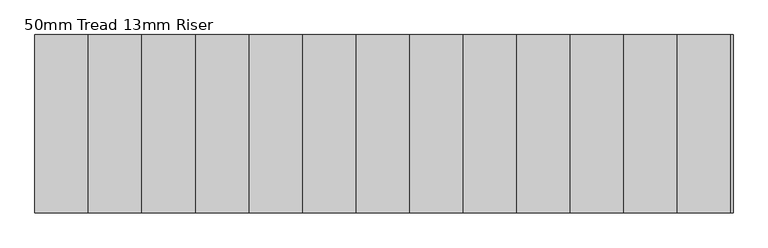
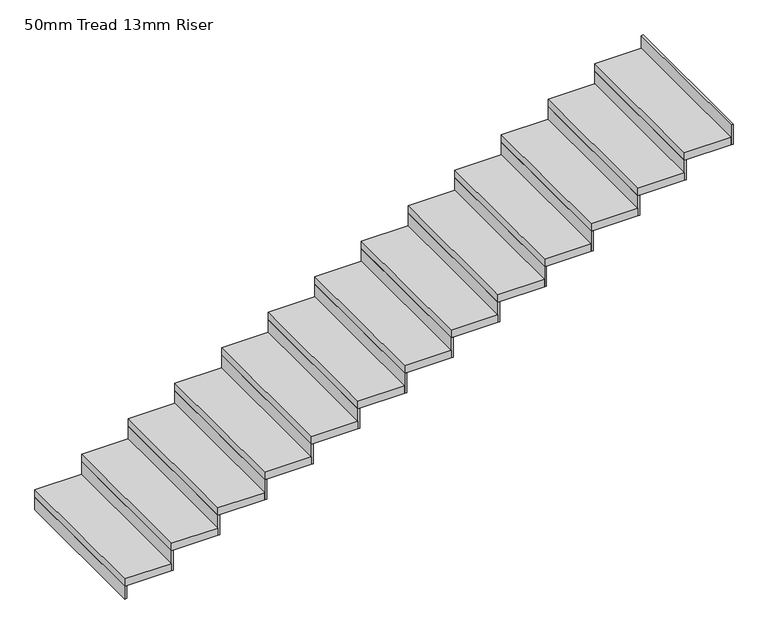
"""IFC4 building model written with IfcOpenShell, lengths in millimetres: stair flight geometry, 50mm Tread 13mm Riser."""

from ifc_helpers import new_model, si_unit, frame, origin, origin_with_axes, place, context, project, spatial, polyline, outline, extrude, source, transform, mapped, element, save


def stair_flight_50mm_tread_13mm_riser_4b704193(model_context):
    return source(origin(), model_context, "Body", "SweptSolid", [
        extrude(outline(polyline([(17862.336337, -4576.2808257), (17849.836337, -4576.2808257), (17849.836337, -3576.2808257), (17862.336337, -3576.2808257), (17862.336337, -4576.2808257)])), origin_with_axes(), (0.0, 0.0, 1.0), 86.3636364),
        extrude(outline(polyline([(18149.836337, -3576.2808257), (18149.836337, -4576.2808257), (17849.836337, -4576.2808257), (17849.836337, -3576.2808257), (18149.836337, -3576.2808257)])), frame((0.0, 0.0, 86.3636364), z_axis=(0.0, 0.0, 1.0), x_axis=(1.0, 0.0, 0.0)), (0.0, 0.0, 1.0), 50.0),
        extrude(outline(polyline([(18162.336337, -4576.2808257), (18149.836337, -4576.2808257), (18149.836337, -3576.2808257), (18162.336337, -3576.2808257), (18162.336337, -4576.2808257)])), frame((0.0, 0.0, 86.3636364), z_axis=(0.0, 0.0, 1.0), x_axis=(1.0, 0.0, 0.0)), (0.0, 0.0, 1.0), 136.3636364),
        extrude(outline(polyline([(18449.836337, -3576.2808257), (18449.836337, -4576.2808257), (18149.836337, -4576.2808257), (18149.836337, -3576.2808257), (18449.836337, -3576.2808257)])), frame((0.0, 0.0, 222.7272727), z_axis=(0.0, 0.0, 1.0), x_axis=(1.0, 0.0, 0.0)), (0.0, 0.0, 1.0), 50.0),
        extrude(outline(polyline([(18462.336337, -4576.2808257), (18449.836337, -4576.2808257), (18449.836337, -3576.2808257), (18462.336337, -3576.2808257), (18462.336337, -4576.2808257)])), frame((0.0, 0.0, 222.7272727), z_axis=(0.0, 0.0, 1.0), x_axis=(1.0, 0.0, 0.0)), (0.0, 0.0, 1.0), 136.3636364),
        extrude(outline(polyline([(18749.836337, -3576.2808257), (18749.836337, -4576.2808257), (18449.836337, -4576.2808257), (18449.836337, -3576.2808257), (18749.836337, -3576.2808257)])), frame((0.0, 0.0, 359.0909091), z_axis=(0.0, 0.0, 1.0), x_axis=(1.0, 0.0, 0.0)), (0.0, 0.0, 1.0), 50.0),
        extrude(outline(polyline([(18762.336337, -4576.2808257), (18749.836337, -4576.2808257), (18749.836337, -3576.2808257), (18762.336337, -3576.2808257), (18762.336337, -4576.2808257)])), frame((0.0, 0.0, 359.0909091), z_axis=(0.0, 0.0, 1.0), x_axis=(1.0, 0.0, 0.0)), (0.0, 0.0, 1.0), 136.3636364),
        extrude(outline(polyline([(19049.836337, -3576.2808257), (19049.836337, -4576.2808257), (18749.836337, -4576.2808257), (18749.836337, -3576.2808257), (19049.836337, -3576.2808257)])), frame((0.0, 0.0, 495.4545455), z_axis=(0.0, 0.0, 1.0), x_axis=(1.0, 0.0, 0.0)), (0.0, 0.0, 1.0), 50.0),
        extrude(outline(polyline([(19062.336337, -4576.2808257), (19049.836337, -4576.2808257), (19049.836337, -3576.2808257), (19062.336337, -3576.2808257), (19062.336337, -4576.2808257)])), frame((0.0, 0.0, 495.4545455), z_axis=(0.0, 0.0, 1.0), x_axis=(1.0, 0.0, 0.0)), (0.0, 0.0, 1.0), 136.3636364),
        extrude(outline(polyline([(19349.836337, -3576.2808257), (19349.836337, -4576.2808257), (19049.836337, -4576.2808257), (19049.836337, -3576.2808257), (19349.836337, -3576.2808257)])), frame((0.0, 0.0, 631.8181818), z_axis=(0.0, 0.0, 1.0), x_axis=(1.0, 0.0, 0.0)), (0.0, 0.0, 1.0), 50.0),
        extrude(outline(polyline([(19362.336337, -4576.2808257), (19349.836337, -4576.2808257), (19349.836337, -3576.2808257), (19362.336337, -3576.2808257), (19362.336337, -4576.2808257)])), frame((0.0, 0.0, 631.8181818), z_axis=(0.0, 0.0, 1.0), x_axis=(1.0, 0.0, 0.0)), (0.0, 0.0, 1.0), 136.3636364),
        extrude(outline(polyline([(19649.836337, -3576.2808257), (19649.836337, -4576.2808257), (19349.836337, -4576.2808257), (19349.836337, -3576.2808257), (19649.836337, -3576.2808257)])), frame((0.0, 0.0, 768.1818182), z_axis=(0.0, 0.0, 1.0), x_axis=(1.0, 0.0, 0.0)), (0.0, 0.0, 1.0), 50.0),
        extrude(outline(polyline([(19662.336337, -4576.2808257), (19649.836337, -4576.2808257), (19649.836337, -3576.2808257), (19662.336337, -3576.2808257), (19662.336337, -4576.2808257)])), frame((0.0, 0.0, 768.1818182), z_axis=(0.0, 0.0, 1.0), x_axis=(1.0, 0.0, 0.0)), (0.0, 0.0, 1.0), 136.3636364),
        extrude(outline(polyline([(19949.836337, -3576.2808257), (19949.836337, -4576.2808257), (19649.836337, -4576.2808257), (19649.836337, -3576.2808257), (19949.836337, -3576.2808257)])), frame((0.0, 0.0, 904.5454545), z_axis=(0.0, 0.0, 1.0), x_axis=(1.0, 0.0, 0.0)), (0.0, 0.0, 1.0), 50.0),
        extrude(outline(polyline([(19962.336337, -4576.2808257), (19949.836337, -4576.2808257), (19949.836337, -3576.2808257), (19962.336337, -3576.2808257), (19962.336337, -4576.2808257)])), frame((0.0, 0.0, 904.5454545), z_axis=(0.0, 0.0, 1.0), x_axis=(1.0, 0.0, 0.0)), (0.0, 0.0, 1.0), 136.3636364),
        extrude(outline(polyline([(20249.836337, -3576.2808257), (20249.836337, -4576.2808257), (19949.836337, -4576.2808257), (19949.836337, -3576.2808257), (20249.836337, -3576.2808257)])), frame((0.0, 0.0, 1040.9090909), z_axis=(0.0, 0.0, 1.0), x_axis=(1.0, 0.0, 0.0)), (0.0, 0.0, 1.0), 50.0),
        extrude(outline(polyline([(20262.336337, -4576.2808257), (20249.836337, -4576.2808257), (20249.836337, -3576.2808257), (20262.336337, -3576.2808257), (20262.336337, -4576.2808257)])), frame((0.0, 0.0, 1040.9090909), z_axis=(0.0, 0.0, 1.0), x_axis=(1.0, 0.0, 0.0)), (0.0, 0.0, 1.0), 136.3636364),
        extrude(outline(polyline([(20549.836337, -3576.2808257), (20549.836337, -4576.2808257), (20249.836337, -4576.2808257), (20249.836337, -3576.2808257), (20549.836337, -3576.2808257)])), frame((0.0, 0.0, 1177.2727273), z_axis=(0.0, 0.0, 1.0), x_axis=(1.0, 0.0, 0.0)), (0.0, 0.0, 1.0), 50.0),
        extrude(outline(polyline([(20562.336337, -4576.2808257), (20549.836337, -4576.2808257), (20549.836337, -3576.2808257), (20562.336337, -3576.2808257), (20562.336337, -4576.2808257)])), frame((0.0, 0.0, 1177.2727273), z_axis=(0.0, 0.0, 1.0), x_axis=(1.0, 0.0, 0.0)), (0.0, 0.0, 1.0), 136.3636364),
        extrude(outline(polyline([(20849.836337, -3576.2808257), (20849.836337, -4576.2808257), (20549.836337, -4576.2808257), (20549.836337, -3576.2808257), (20849.836337, -3576.2808257)])), frame((0.0, 0.0, 1313.6363636), z_axis=(0.0, 0.0, 1.0), x_axis=(1.0, 0.0, 0.0)), (0.0, 0.0, 1.0), 50.0),
        extrude(outline(polyline([(20862.336337, -4576.2808257), (20849.836337, -4576.2808257), (20849.836337, -3576.2808257), (20862.336337, -3576.2808257), (20862.336337, -4576.2808257)])), frame((0.0, 0.0, 1313.6363636), z_axis=(0.0, 0.0, 1.0), x_axis=(1.0, 0.0, 0.0)), (0.0, 0.0, 1.0), 136.3636364),
        extrude(outline(polyline([(21149.836337, -3576.2808257), (21149.836337, -4576.2808257), (20849.836337, -4576.2808257), (20849.836337, -3576.2808257), (21149.836337, -3576.2808257)])), frame((0.0, 0.0, 1450.0), z_axis=(0.0, 0.0, 1.0), x_axis=(1.0, 0.0, 0.0)), (0.0, 0.0, 1.0), 50.0),
        extrude(outline(polyline([(21162.336337, -4576.2808257), (21149.836337, -4576.2808257), (21149.836337, -3576.2808257), (21162.336337, -3576.2808257), (21162.336337, -4576.2808257)])), frame((0.0, 0.0, 1450.0), z_axis=(0.0, 0.0, 1.0), x_axis=(1.0, 0.0, 0.0)), (0.0, 0.0, 1.0), 136.3636364),
        extrude(outline(polyline([(21449.836337, -3576.2808257), (21449.836337, -4576.2808257), (21149.836337, -4576.2808257), (21149.836337, -3576.2808257), (21449.836337, -3576.2808257)])), frame((0.0, 0.0, 1586.3636364), z_axis=(0.0, 0.0, 1.0), x_axis=(1.0, 0.0, 0.0)), (0.0, 0.0, 1.0), 50.0),
        extrude(outline(polyline([(21462.336337, -4576.2808257), (21449.836337, -4576.2808257), (21449.836337, -3576.2808257), (21462.336337, -3576.2808257), (21462.336337, -4576.2808257)])), frame((0.0, 0.0, 1586.3636364), z_axis=(0.0, 0.0, 1.0), x_axis=(1.0, 0.0, 0.0)), (0.0, 0.0, 1.0), 136.3636364),
        extrude(outline(polyline([(21762.336337, -4576.2808257), (21749.836337, -4576.2808257), (21749.836337, -3576.2808257), (21762.336337, -3576.2808257), (21762.336337, -4576.2808257)])), frame((0.0, 0.0, 1722.7272727), z_axis=(0.0, 0.0, 1.0), x_axis=(1.0, 0.0, 0.0)), (0.0, 0.0, 1.0), 136.3636364),
        extrude(outline(polyline([(21749.836337, -3576.2808257), (21749.836337, -4576.2808257), (21449.836337, -4576.2808257), (21449.836337, -3576.2808257), (21749.836337, -3576.2808257)])), frame((0.0, 0.0, 1722.7272727), z_axis=(0.0, 0.0, 1.0), x_axis=(1.0, 0.0, 0.0)), (0.0, 0.0, 1.0), 50.0),
    ])


if __name__ == "__main__":
    model = new_model("IFC4")
    model_context = context("Model", 3, world=origin())
    ifc_project = project(units=[si_unit("LENGTHUNIT", "METRE", prefix="MILLI")], contexts=[model_context])
    site = spatial("IfcSite", under=ifc_project)
    building = spatial("IfcBuilding", under=site)
    placement = place(None, origin())
    stair_flight_50mm_tread_13mm_riser_shape = stair_flight_50mm_tread_13mm_riser_4b704193(model_context)
    element("IfcStairFlight", 1, ObjectType="50mm Tread 13mm Riser", at=placement, inside=building, context=model_context, shape_type="MappedRepresentation", body=[
        mapped(stair_flight_50mm_tread_13mm_riser_shape, transform((0.0, 0.0, 0.0), x_axis=(1.0, 0.0, 0.0), y_axis=(0.0, 1.0, 0.0), z_axis=(0.0, 0.0, 1.0))),
    ])
    save(model, "model.ifc")
